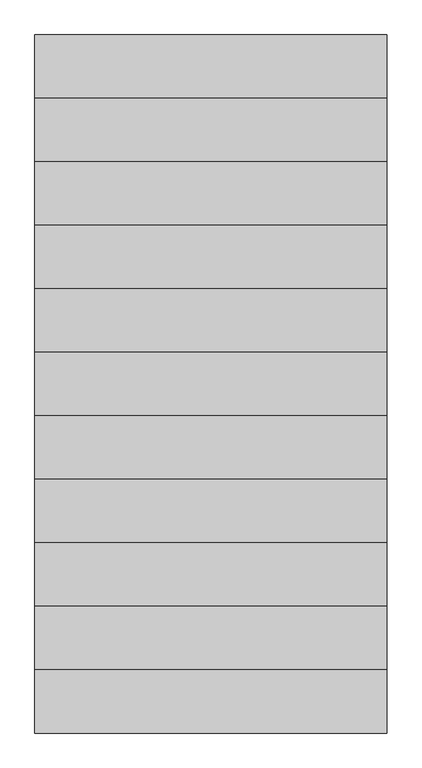
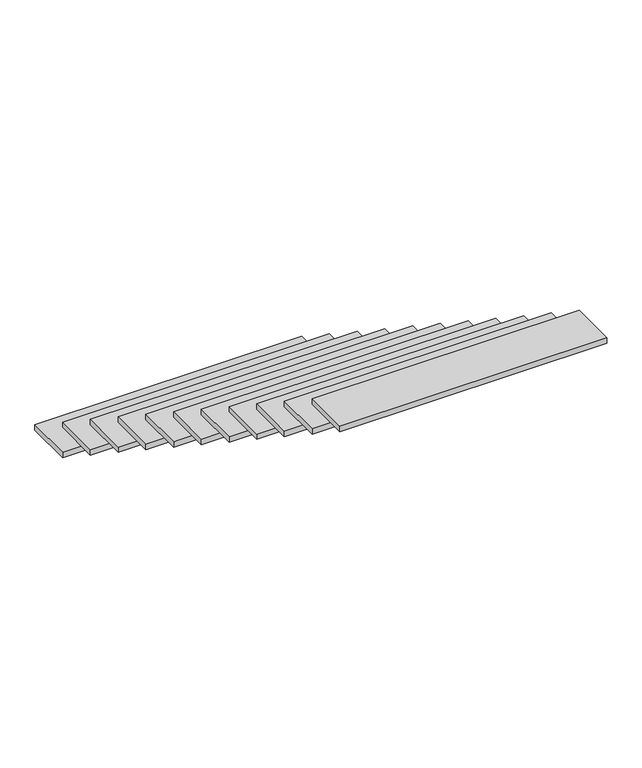
"""IFC4 building model written with IfcOpenShell, lengths in millimetres: stair flight geometry."""

from ifc_helpers import new_model, si_unit, frame, origin, place, context, project, spatial, polyline, outline, extrude, source, transform, mapped, element, save


def stair_flight_5b252c62(model_context):
    return source(origin(), model_context, "Body", "SweptSolid", [
        extrude(outline(polyline([(16085.3403387, 4647.6066446), (14585.3403387, 4647.6066446), (14585.3403387, 4917.6066446), (16085.3403387, 4917.6066446), (16085.3403387, 4647.6066446)])), frame((0.0, 0.0, 9998.7692308), z_axis=(0.0, 0.0, 1.0), x_axis=(1.0, 0.0, 0.0)), (0.0, 0.0, 1.0), 32.0),
        extrude(outline(polyline([(16085.3403387, 4377.6066446), (14585.3403387, 4377.6066446), (14585.3403387, 4647.6066446), (16085.3403387, 4647.6066446), (16085.3403387, 4377.6066446)])), frame((0.0, 0.0, 10177.8901099), z_axis=(0.0, 0.0, 1.0), x_axis=(1.0, 0.0, 0.0)), (0.0, 0.0, 1.0), 32.0),
        extrude(outline(polyline([(16085.3403387, 4107.6066446), (14585.3403387, 4107.6066446), (14585.3403387, 4377.6066446), (16085.3403387, 4377.6066446), (16085.3403387, 4107.6066446)])), frame((0.0, 0.0, 10357.010989), z_axis=(0.0, 0.0, 1.0), x_axis=(1.0, 0.0, 0.0)), (0.0, 0.0, 1.0), 32.0),
        extrude(outline(polyline([(16085.3403387, 3837.6066446), (14585.3403387, 3837.6066446), (14585.3403387, 4107.6066446), (16085.3403387, 4107.6066446), (16085.3403387, 3837.6066446)])), frame((0.0, 0.0, 10536.1318681), z_axis=(0.0, 0.0, 1.0), x_axis=(1.0, 0.0, 0.0)), (0.0, 0.0, 1.0), 32.0),
        extrude(outline(polyline([(16085.3403387, 3567.6066446), (14585.3403387, 3567.6066446), (14585.3403387, 3837.6066446), (16085.3403387, 3837.6066446), (16085.3403387, 3567.6066446)])), frame((0.0, 0.0, 10715.2527473), z_axis=(0.0, 0.0, 1.0), x_axis=(1.0, 0.0, 0.0)), (0.0, 0.0, 1.0), 32.0),
        extrude(outline(polyline([(16085.3403387, 3297.6066446), (14585.3403387, 3297.6066446), (14585.3403387, 3567.6066446), (16085.3403387, 3567.6066446), (16085.3403387, 3297.6066446)])), frame((0.0, 0.0, 10894.3736264), z_axis=(0.0, 0.0, 1.0), x_axis=(1.0, 0.0, 0.0)), (0.0, 0.0, 1.0), 32.0),
        extrude(outline(polyline([(16085.3403387, 3027.6066446), (14585.3403387, 3027.6066446), (14585.3403387, 3297.6066446), (16085.3403387, 3297.6066446), (16085.3403387, 3027.6066446)])), frame((0.0, 0.0, 11073.4945055), z_axis=(0.0, 0.0, 1.0), x_axis=(1.0, 0.0, 0.0)), (0.0, 0.0, 1.0), 32.0),
        extrude(outline(polyline([(16085.3403387, 2757.6066446), (14585.3403387, 2757.6066446), (14585.3403387, 3027.6066446), (16085.3403387, 3027.6066446), (16085.3403387, 2757.6066446)])), frame((0.0, 0.0, 11252.6153846), z_axis=(0.0, 0.0, 1.0), x_axis=(1.0, 0.0, 0.0)), (0.0, 0.0, 1.0), 32.0),
        extrude(outline(polyline([(16085.3403387, 2487.6066446), (14585.3403387, 2487.6066446), (14585.3403387, 2757.6066446), (16085.3403387, 2757.6066446), (16085.3403387, 2487.6066446)])), frame((0.0, 0.0, 11431.7362637), z_axis=(0.0, 0.0, 1.0), x_axis=(1.0, 0.0, 0.0)), (0.0, 0.0, 1.0), 32.0),
        extrude(outline(polyline([(16085.3403387, 2217.6066446), (14585.3403387, 2217.6066446), (14585.3403387, 2487.6066446), (16085.3403387, 2487.6066446), (16085.3403387, 2217.6066446)])), frame((0.0, 0.0, 11610.8571429), z_axis=(0.0, 0.0, 1.0), x_axis=(1.0, 0.0, 0.0)), (0.0, 0.0, 1.0), 32.0),
        extrude(outline(polyline([(16085.3403387, 1947.6066446), (14585.3403387, 1947.6066446), (14585.3403387, 2217.6066446), (16085.3403387, 2217.6066446), (16085.3403387, 1947.6066446)])), frame((0.0, 0.0, 11789.978022), z_axis=(0.0, 0.0, 1.0), x_axis=(1.0, 0.0, 0.0)), (0.0, 0.0, 1.0), 32.0),
    ])


if __name__ == "__main__":
    model = new_model("IFC4")
    model_context = context("Model", 3, world=origin())
    ifc_project = project(units=[si_unit("LENGTHUNIT", "METRE", prefix="MILLI")], contexts=[model_context])
    site = spatial("IfcSite", under=ifc_project)
    building = spatial("IfcBuilding", under=site)
    placement = place(None, origin())
    stair_flight_shape = stair_flight_5b252c62(model_context)
    element("IfcStairFlight", 1, at=placement, inside=building, context=model_context, shape_type="MappedRepresentation", body=[
        mapped(stair_flight_shape, transform((0.0, 0.0, 0.0), x_axis=(1.0, 0.0, 0.0), y_axis=(0.0, 1.0, 0.0), z_axis=(0.0, 0.0, 1.0))),
    ])
    save(model, "model.ifc")

# Revit data of these elements
# Element 1 (IfcStairFlight)
#   Materials on its faces: "철강"
# Materials
#   "철강": class "Generic", colour RGB 143 142 141, transparency 0, Description = "철골+가공조립+세우기", Cost = 0
